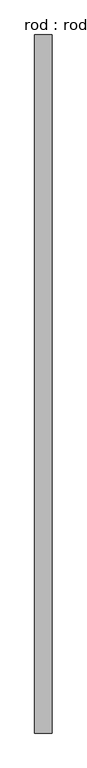
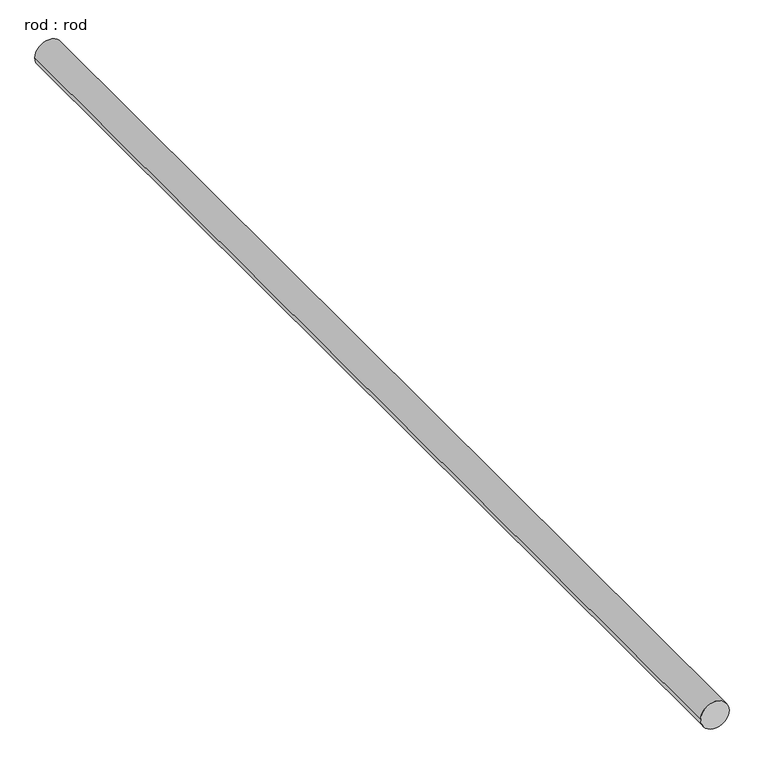
"""IFC4 building model written with IfcOpenShell, lengths in millimetres: proxy geometry, rod : rod."""

from ifc_helpers import new_model, si_unit, point, frame, frame_2d, origin, place, context, project, spatial, circle_curve, trimmed, segment, composite_curve, outline, extrude, source, transform, mapped, element, save


def rod_rod_7f8ae2a6(model_context):
    return source(origin(), model_context, "Body", "SweptSolid", [
        extrude(outline(composite_curve([segment(trimmed(circle_curve(frame_2d((0.0108462, 0.0)), 200.0), [point((0.0108462, 200.0))], [point((0.0108462, -200.0))], False, "CARTESIAN"), True, "CONTINUOUS"), segment(trimmed(circle_curve(frame_2d((0.0108462, 0.0)), 200.0), [point((0.0108462, -200.0))], [point((0.0108462, 200.0))], False, "CARTESIAN"), True, "CONTINUOUS")], self_intersect=False)), frame((0.0, -4022.6614708, 0.0), z_axis=(0.0, 1.0, 0.0), x_axis=(0.0, 0.0, 1.0)), (0.0, 0.0, 1.0), 16230.7801723),
    ])


if __name__ == "__main__":
    model = new_model("IFC4")
    model_context = context("Model", 3, world=origin())
    ifc_project = project(units=[si_unit("LENGTHUNIT", "METRE", prefix="MILLI")], contexts=[model_context])
    site = spatial("IfcSite", under=ifc_project)
    building = spatial("IfcBuilding", under=site)
    placement = place(None, origin())
    rod_rod_shape = rod_rod_7f8ae2a6(model_context)
    element("IfcBuildingElementProxy", 1, Name="rod : rod", ObjectType="rod : rod", at=placement, inside=building, context=model_context, shape_type="MappedRepresentation", body=[
        mapped(rod_rod_shape, transform((0.0, 0.0, 0.0), x_axis=(1.0, 0.0, 0.0), y_axis=(0.0, 1.0, 0.0), z_axis=(0.0, 0.0, 1.0))),
    ])
    save(model, "model.ifc")

# Revit data of these elements
# Type "rod : rod"
#   Default Elevation = 0
